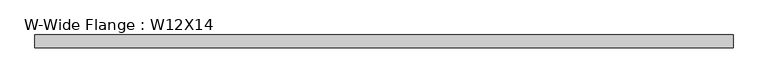
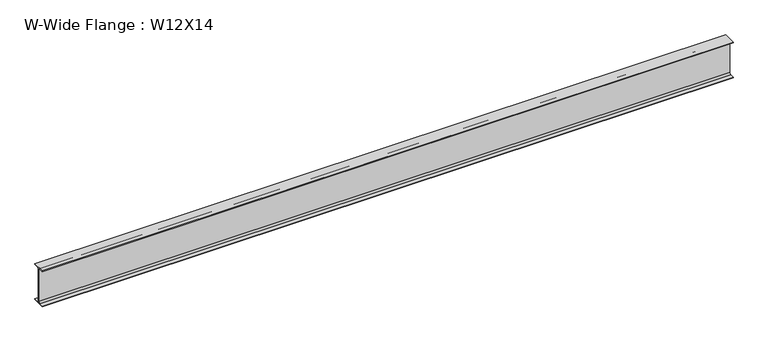
"""IFC4 building model written with IfcOpenShell, lengths in millimetres: beam geometry, W-Wide Flange : W12X14."""

from ifc_helpers import new_model, si_unit, point, frame, frame_2d, origin, place, context, project, spatial, polyline, circle_curve, trimmed, segment, composite_curve, outline, extrude, source, transform, mapped, element, save


def w_wide_flange_w12x14_cdfe6272(model_context):
    return source(origin(), model_context, "Body", "SweptSolid", [
        extrude(outline(composite_curve([segment(polyline([(50.419, -145.415), (50.419, -151.13), (-50.419, -151.13), (-50.419, -145.415), (-15.875, -145.415)]), True, "CONTINUOUS"), segment(trimmed(circle_curve(frame_2d((-15.875, -132.08)), 13.335), [point((-15.875, -145.415))], [point((-2.54, -132.08))], True, "CARTESIAN"), True, "CONTINUOUS"), segment(polyline([(-2.54, -132.08), (-2.54, 132.08)]), True, "CONTINUOUS"), segment(trimmed(circle_curve(frame_2d((-15.875, 132.08)), 13.335), [point((-2.54, 132.08))], [point((-15.875, 145.415))], True, "CARTESIAN"), True, "CONTINUOUS"), segment(polyline([(-15.875, 145.415), (-50.419, 145.415), (-50.419, 151.13), (50.419, 151.13), (50.419, 145.415), (15.875, 145.415)]), True, "CONTINUOUS"), segment(trimmed(circle_curve(frame_2d((15.875, 132.08)), 13.335), [point((15.875, 145.415))], [point((2.54, 132.08))], True, "CARTESIAN"), True, "CONTINUOUS"), segment(polyline([(2.54, 132.08), (2.54, -132.08)]), True, "CONTINUOUS"), segment(trimmed(circle_curve(frame_2d((15.875, -132.08)), 13.335), [point((2.54, -132.08))], [point((15.875, -145.415))], True, "CARTESIAN"), True, "CONTINUOUS"), segment(polyline([(15.875, -145.415), (50.419, -145.415)]), True, "CONTINUOUS")], self_intersect=False)), frame((-2743.327, 0.0, 0.0), z_axis=(1.0, 0.0, 0.0), x_axis=(0.0, 1.0, 0.0)), (0.0, 0.0, 1.0), 5524.5),
    ])


if __name__ == "__main__":
    model = new_model("IFC4")
    model_context = context("Model", 3, world=origin())
    ifc_project = project(units=[si_unit("LENGTHUNIT", "METRE", prefix="MILLI")], contexts=[model_context])
    site = spatial("IfcSite", under=ifc_project)
    building = spatial("IfcBuilding", under=site)
    placement = place(None, origin())
    w_wide_flange_w12x14_shape = w_wide_flange_w12x14_cdfe6272(model_context)
    element("IfcBeam", 1, ObjectType="W-Wide Flange : W12X14", at=placement, inside=building, context=model_context, shape_type="MappedRepresentation", body=[
        mapped(w_wide_flange_w12x14_shape, transform((0.0, 0.0, 0.0), x_axis=(1.0, 0.0, 0.0), y_axis=(0.0, 1.0, 0.0), z_axis=(0.0, 0.0, 1.0))),
    ])
    save(model, "model.ifc")

# Revit data of these elements
# Type "W-Wide Flange : W12X14"
#   Assembly Code = "B10"
#   W = 14
#   Length [instance default] = 5' - 0"
#   bf = 0' - 3.97"
#   d = 0' - 11.9"
#   k = 0' - 0 3/4"
#   k2 = 0' - 0.525"
#   tf = 0' - 0.225"
#   tw = 0' - 0.2"
#   A = 0.0288889 SF
#   Structural Material [instance default] = Steel ASTM A992
# Element 1 (IfcBeam, "W-Wide Flange : W12X14")
#   Materials on its faces: "Steel ASTM A992"
# Materials
#   "Steel ASTM A992": class "Metal", colour RGB 199 199 199, transparency 0, Description = "Structural steel 50ksi", Cost = 0
